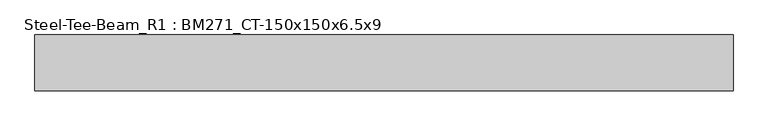
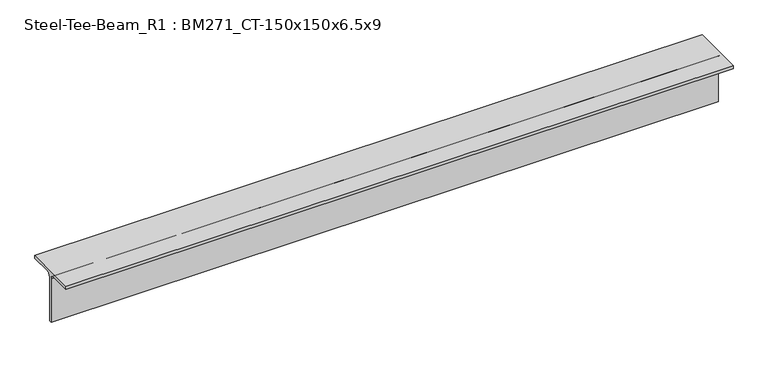
"""IFC4 building model written with IfcOpenShell, lengths in millimetres: member geometry, Steel-Tee-Beam_R1 : BM271_CT-150x150x6.5x9."""

from ifc_helpers import new_model, si_unit, point, frame, frame_2d, origin, place, context, project, spatial, polyline, circle_curve, trimmed, segment, composite_curve, outline, extrude, source, transform, mapped, element, save


def steel_tee_beam_r1_bm271_ct_150x150x6_5x9_c9def017(model_context):
    return source(origin(), model_context, "Body", "SweptSolid", [
        extrude(outline(composite_curve([segment(polyline([(75.0, 75.0), (75.0, 66.0), (16.25, 66.0)]), True, "CONTINUOUS"), segment(trimmed(circle_curve(frame_2d((16.25, 53.0)), 13.0), [point((16.25, 66.0))], [point((3.25, 53.0))], True, "CARTESIAN"), True, "CONTINUOUS"), segment(polyline([(3.25, 53.0), (3.25, -75.0), (-3.25, -75.0), (-3.25, 53.0)]), True, "CONTINUOUS"), segment(trimmed(circle_curve(frame_2d((-16.25, 53.0)), 13.0), [point((-3.25, 53.0))], [point((-16.25, 66.0))], True, "CARTESIAN"), True, "CONTINUOUS"), segment(polyline([(-16.25, 66.0), (-75.0, 66.0), (-75.0, 75.0), (75.0, 75.0)]), True, "CONTINUOUS")], self_intersect=False)), frame((-1113.6541462, 0.0, 0.0), z_axis=(1.0, 0.0, 0.0), x_axis=(0.0, 1.0, 0.0)), (0.0, 0.0, 1.0), 1868.963443),
    ])


if __name__ == "__main__":
    model = new_model("IFC4")
    model_context = context("Model", 3, world=origin())
    ifc_project = project(units=[si_unit("LENGTHUNIT", "METRE", prefix="MILLI")], contexts=[model_context])
    site = spatial("IfcSite", under=ifc_project)
    building = spatial("IfcBuilding", under=site)
    placement = place(None, origin())
    steel_tee_beam_r1_bm271_ct_150x150x6_5x9_shape = steel_tee_beam_r1_bm271_ct_150x150x6_5x9_c9def017(model_context)
    element("IfcMember", 1, ObjectType="Steel-Tee-Beam_R1 : BM271_CT-150x150x6.5x9", at=placement, inside=building, context=model_context, shape_type="MappedRepresentation", body=[
        mapped(steel_tee_beam_r1_bm271_ct_150x150x6_5x9_shape, transform((0.0, 0.0, 0.0), x_axis=(1.0, 0.0, 0.0), y_axis=(0.0, 1.0, 0.0), z_axis=(0.0, 0.0, 1.0))),
    ])
    save(model, "model.ifc")

# Revit data of these elements
# Type "Steel-Tee-Beam_R1 : BM271_CT-150x150x6.5x9"
#   Keynote = "CT-150x150x6.5x9"
#   Surface Area = 0.588841 m²/m
#   Section Area = 23.3904 cm²
#   Mass per Unit Length = 18.3614 kg/m
#   Length [instance default] = 1.5240 m
#   bf = 0.1500 m
#   d = 0.1500 m
#   k = 0.0220 m
#   r = 0.0130 m
#   tf = 0.0090 m
#   tw = 0.0065 m
#   hec_material4 [instance default] = none
#   hec_material3 [instance default] = none
#   hec_material2 [instance default] = none
#   hec_material1 [instance default] = none
#   Structural Material [instance default] = Steel, 45-345
#   Assembly Code = ""
# Element 1 (IfcMember, "Steel-Tee-Beam_R1 : BM271_CT-150x150x6.5x9")
#   Structural Material = none
# Materials
#   "Steel, 45-345": class "Metal", colour RGB 189 187 185, transparency 0, Description = "Steel 345 MPa", Cost = 0
